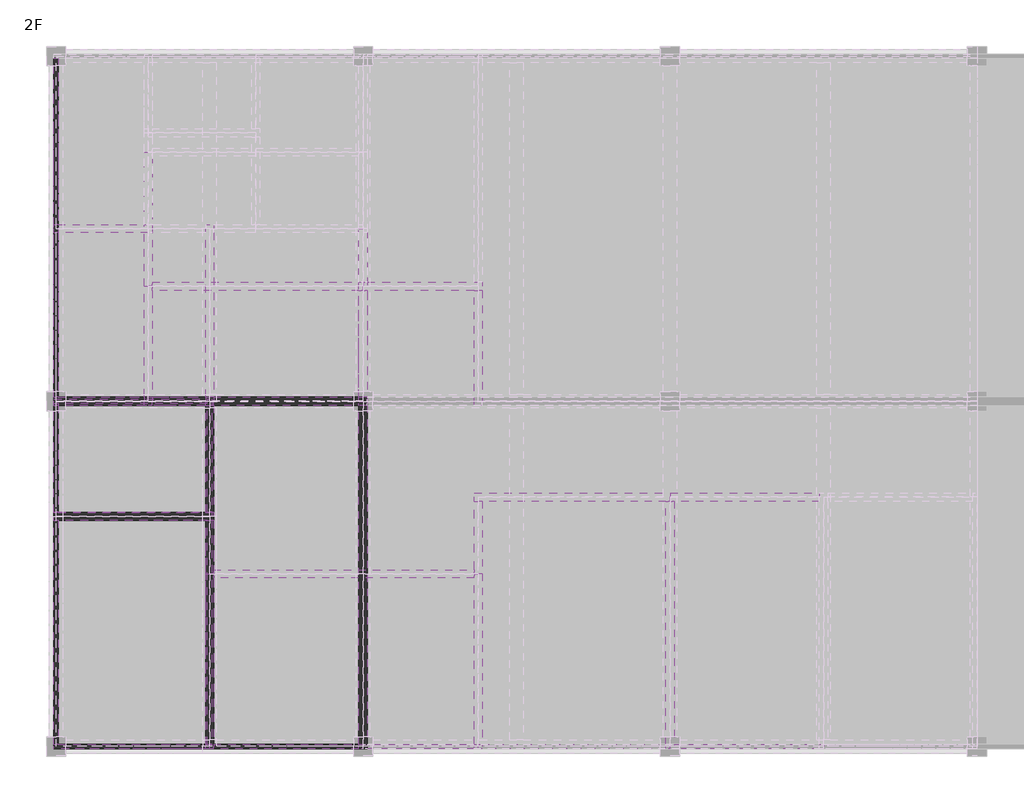
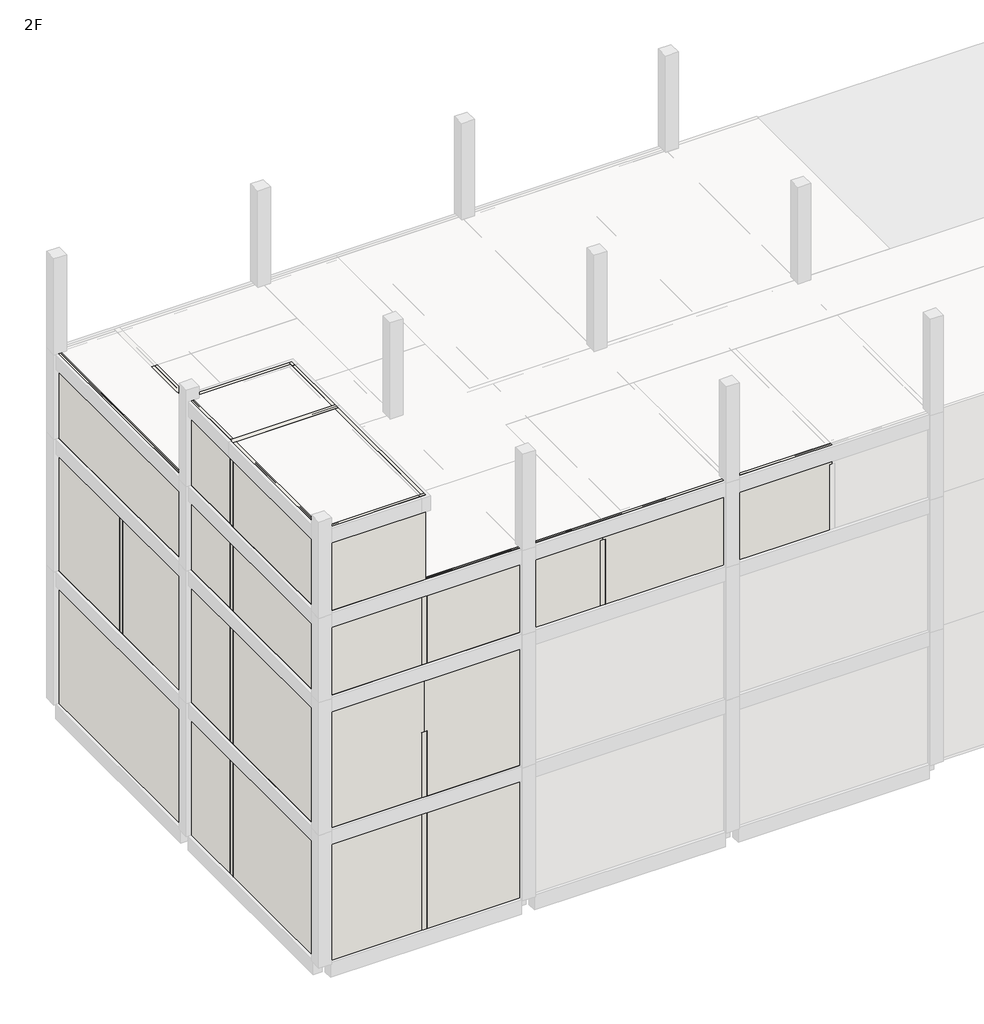
# One storey, part 1 of 7: 58 walls.
# Revit data of these elements (continued)
# Materials (continued)
#   "A04AK073-00001_Concrete Brick_0.5B": class "Concrete", colour RGB 180 180 180, transparency 0, Description = "Conc. Block", W00) Work Master Code = "A04AK073-00001", W01) Work Master_Lv1 = "Finishing Work", W02) Work Master_Lv2 = "Masonry Work", W03) Work Master_Spec.1 = "Concrete Brick", W04) Work Master_Spec.2 = "[0.5B] w/ All Reinf.(Lath, Steel Tie, Anchor Bar, Mortar, ETC.), Filler, Sealant, Lintel/Sill for Opening, ETC.", Cost = 0
#   "A04AS164-00002_Plastering_Int": class "Concrete", colour RGB 183 186 184, transparency 0, Description = "LATEX PAINT ON THK.15 CEMENT PLASTER", W00) Work Master Code = "A04AS164-00002", W01) Work Master_Lv1 = "Finishing Work", W02) Work Master_Lv2 = "Plastering Work", W03) Work Master_Spec.1 = "Plastering", W04) Work Master_Spec.2 = "for Internal Masonry Wall", Cost = 0
#   "A04AL078-00002_Int Wall Painting_Water Emulsion Paint": class "Finish", colour RGB 128 128 64, transparency 0, Description = "Plastic", W00) Work Master Code = "A04AL078-00002", W01) Work Master_Lv1 = "Finishing Work", W02) Work Master_Lv2 = "Painting Work", W03) Work Master_Spec.1 = "Internal Wall Painting", W04) Work Master_Spec.2 = "Water Emulsion Paint", Cost = 0
#   "A04AK069-00002_Reinforced Concrete Block_THK 100-200mm": class "Concrete", colour RGB 180 180 180, transparency 0, Description = "Conc. Block", W00) Work Master Code = "A04AK069-00002", W01) Work Master_Lv1 = "Finishing Work", W02) Work Master_Lv2 = "Masonry Work", W03) Work Master_Spec.1 = "Reinforced Concrete Block", W04) Work Master_Spec.2 = "w/ All Reinf.(Lath, Steel Tie, Anchor Bar, Mortar, ETC.), Filler, Sealant, Lintel/Sill for Opening, ETC.", W05) Work Master_Spec.3 = "100mm<THK≤200mm", Cost = 0
#   "Default Wall": class "Miscellaneous", colour RGB 80 80 80, transparency 0
# Room at (79959.652, 167173.861) mm, phase "New Construction", upper offset 2700 mm, lower offset 0 mm
#   Department = "AR"
#   Base Finish = "WK3"
#   Ceiling Finish = "CL3"
#   Wall Finish = "IW5"
#   Floor Finish = "FL2"
#   Number = "4.5"
#   Name = "Office-1"
#   Interior Finish = "IW5..N/A..N/A,,WK3..N/A,,FL2..N/A,,CL3..N/A"
#   Exterior Finish = "RF1..N/A,,EW2..N/A..N/A"
# Room at (84959.652, 167173.861) mm, phase "New Construction", upper offset 3500 mm, lower offset 0 mm
#   Department = "FF"
#   Base Finish = "WK1"
#   Ceiling Finish = ""
#   Wall Finish = "IW5"
#   Floor Finish = "FL1"
#   Number = "4.6"
#   Name = "Fire Gas Room"
#   Interior Finish = "IW5..N/A..N/A,,WK1..N/A,,FL1..N/A,,N/A..N/A"
#   Exterior Finish = "RF1..N/A,,EW2..N/A..N/A"
# Room at (78709.652, 174423.861) mm, phase "New Construction", upper offset 2700 mm, lower offset 0 mm
#   Department = "AR"
#   Base Finish = "WK3"
#   Ceiling Finish = "CL3"
#   Wall Finish = "IW5"
#   Floor Finish = "FL2"
#   Number = "4.7"
#   Name = "Document Room"
#   Interior Finish = "IW5..N/A..N/A,,WK3..N/A,,FL2..N/A,,CL3..N/A"
#   Exterior Finish = "RF1..N/A,,N/A..N/A..N/A"
# Room at (58959.652, 167173.861) mm, phase "New Construction", upper offset 2700 mm, lower offset 0 mm
#   Department = "AR"
#   Base Finish = "WK3"
#   Ceiling Finish = "CL3"
#   Wall Finish = "IW5"
#   Floor Finish = "FL2"
#   Number = "4.8"
#   Name = "Storage"
#   Interior Finish = "IW5..N/A..N/A,,WK3..N/A,,FL2..N/A,,CL3..N/A"
#   Exterior Finish = "RF1..N/A,,EW1..N/A..N/A"
# Room at (52959.652, 166173.861) mm, phase "New Construction", upper offset 2700 mm, lower offset 0 mm
#   Department = "AR"
#   Base Finish = "WK3"
#   Ceiling Finish = "CL3"
#   Wall Finish = "IW5"
#   Floor Finish = "FL2"
#   Number = "4.9"
#   Name = "Break Room"
#   Interior Finish = "IW5..N/A..N/A,,WK3..N/A,,FL2..N/A,,CL3..N/A"
#   Exterior Finish = "RF1..N/A,,EW2..N/A..N/A"
# Room at (50659.652, 177673.861) mm, phase "New Construction", upper offset 2700 mm, lower offset 0 mm
#   Department = "AR"
#   Base Finish = ""
#   Ceiling Finish = "CL4"
#   Wall Finish = "IW3"
#   Floor Finish = "FL3"
#   Number = "4.10"
#   Name = "Toilet"
#   Interior Finish = "IW3..N/A..N/A,,N/A..N/A,,FL3..N/A,,CL4..N/A"
#   Exterior Finish = "RF1..N/A,,N/A..N/A..N/A"
# Room at (50659.652, 180673.861) mm, phase "New Construction", upper offset 2700 mm, lower offset 0 mm
#   Department = "AR"
#   Base Finish = ""
#   Ceiling Finish = "CL4"
#   Wall Finish = "IW3"
#   Floor Finish = "FL3"
#   Number = "4.11"
#   Name = "Shower"
#   Interior Finish = "IW3..N/A..N/A,,N/A..N/A,,FL3..N/A,,CL4..N/A"
#   Exterior Finish = "RF1..N/A,,EW2..N/A..N/A"
# Room at (61459.652, 177423.861) mm, phase "New Construction", upper offset 5500 mm, lower offset 0 mm
#   Department = "CI"
#   Base Finish = "WK1"
#   Ceiling Finish = "CL1"
#   Wall Finish = "IW5"
#   Floor Finish = "FL1"
#   Number = "2.0"
#   Name = "Electrical Room-1"
#   Interior Finish = "IW5..N/A..N/A,,WK1..N/A,,FL1..N/A,,CL1..N/A"
#   Exterior Finish = "N/A..N/A,,EW1..EW2..N/A"
# Room at (70459.652, 168423.861) mm, phase "New Construction", upper offset 5500 mm, lower offset 0 mm
#   Department = "EL"
#   Base Finish = "WK1"
#   Ceiling Finish = "CL1"
#   Wall Finish = "IW5"
#   Floor Finish = "FL1"
#   Number = "2.1"
#   Name = "Electrical Room-2"
#   Interior Finish = "IW5..N/A..N/A,,WK1..N/A,,FL1..N/A,,CL1..N/A"
#   Exterior Finish = "N/A..N/A,,EW1..EW2..N/A"
# Room at (82459.652, 177423.861) mm, phase "New Construction", upper offset 5500 mm, lower offset 0 mm
#   Department = "AR"
#   Base Finish = "WK1"
#   Ceiling Finish = "CL1"
#   Wall Finish = "IW5"
#   Floor Finish = "FL1"
#   Number = "2.2"
#   Name = "Electrical Room (GIS)"
#   Interior Finish = "IW5..N/A..N/A,,WK1..N/A,,FL1..N/A,,CL1..N/A"
#   Exterior Finish = "N/A..N/A,,EW1..EW2..N/A"
# Room at (51459.652, 168423.861) mm, phase "New Construction", upper offset 2700 mm, lower offset 0 mm
#   Department = "AR"
#   Base Finish = "WK3"
#   Ceiling Finish = "CL3"
#   Wall Finish = "IW5"
#   Floor Finish = "FL2"
#   Number = "2.3"
#   Name = "Lobby"
#   Interior Finish = "IW5..N/A..N/A,,WK3..N/A,,FL2..N/A,,CL3..N/A"
#   Exterior Finish = "N/A..N/A,,EW2..N/A..N/A"
# Room at (47459.652, 171423.861) mm, phase "New Construction", upper offset 5500 mm, lower offset 0 mm
#   Department = "PATHV2"
#   Base Finish = ""
#   Ceiling Finish = ""
#   Wall Finish = ""
#   Floor Finish = ""
#   Number = "2.4"
#   Name = "Elevator"
#   Interior Finish = "N/A..N/A..N/A,,N/A..N/A,,N/A..N/A,,N/A..N/A"
#   Exterior Finish = "N/A..N/A,,EW2..N/A..N/A"
# Room at (47459.652, 166923.861) mm, phase "New Construction", upper offset 5500 mm, lower offset 0 mm
#   Department = "PATHV1"
#   Base Finish = "WK3"
#   Ceiling Finish = "CL1"
#   Wall Finish = "IW5"
#   Floor Finish = "FL2"
#   Number = "2.5"
#   Name = "Staircase"
#   Interior Finish = "IW5..N/A..N/A,,WK3..N/A,,FL2..N/A,,CL1..N/A"
#   Exterior Finish = "N/A..N/A,,EW2..N/A..N/A"
# Room at (65459.652, 177423.861) mm, phase "New Construction", upper offset 3400 mm, lower offset 0 mm
#   Department = "CI"
#   Base Finish = ""
#   Ceiling Finish = "CL3"
#   Wall Finish = "IW5"
#   Floor Finish = "FL5"
#   Number = "3.0"
#   Name = "Central Control Room"
#   Interior Finish = "IW5..N/A..N/A,,N/A..N/A,,FL5..N/A,,CL3..N/A"
#   Exterior Finish = "N/A..N/A,,EW1..N/A..N/A"
# Room at (65459.652, 168423.861) mm, phase "New Construction", upper offset 3000 mm, lower offset 0 mm
#   Department = "CI"
#   Base Finish = ""
#   Ceiling Finish = "CL3"
#   Wall Finish = "IW5"
#   Floor Finish = "FL5"
#   Number = "3.1"
#   Name = "Electronic Room"
#   Interior Finish = "IW5..N/A..N/A,,N/A..N/A,,FL5..N/A,,CL3..N/A"
#   Exterior Finish = "N/A..N/A,,EW1..N/A..N/A"
# Room at (80959.652, 180173.861) mm, phase "New Construction", upper offset 2700 mm, lower offset 0 mm
#   Department = "AR"
#   Base Finish = ""
#   Ceiling Finish = "CL3"
#   Wall Finish = "IW5"
#   Floor Finish = "FL5"
#   Number = "3.2"
#   Name = "Computer Room"
#   Interior Finish = "IW5..N/A..N/A,,N/A..N/A,,FL5..N/A,,CL3..N/A"
#   Exterior Finish = "N/A..N/A,,EW2..N/A..N/A"
# Room at (82459.652, 168423.861) mm, phase "New Construction", upper offset 5500 mm, lower offset 0 mm
#   Department = "EL"
#   Base Finish = ""
#   Ceiling Finish = "CL3"
#   Wall Finish = "IW5"
#   Floor Finish = "FL5"
#   Number = "3.3"
#   Name = "Electrical Room -3"
#   Interior Finish = "IW5..N/A..N/A,,N/A..N/A,,FL5,,CL3..N/A"
#   Exterior Finish = "N/A..N/A,,EW2..N/A..N/A"
# Room at (80959.652, 174673.861) mm, phase "New Construction", upper offset 2700 mm, lower offset 0 mm
#   Department = "CI"
#   Base Finish = ""
#   Ceiling Finish = "CL3"
#   Wall Finish = "IW5"
#   Floor Finish = "FL5"
#   Number = "3.4"
#   Name = "Communication Room"
#   Interior Finish = "IW5..N/A..N/A,,N/A..N/A,,FL5..N/A,,CL3..N/A"
#   Exterior Finish = "N/A..N/A,,N/A..N/A..N/A"
# Room at (46659.652, 179673.861) mm, phase "New Construction", upper offset 5500 mm, lower offset 0 mm
#   Department = "PATHV3"
#   Base Finish = ""
#   Ceiling Finish = ""
#   Wall Finish = ""
#   Floor Finish = ""
#   Number = "3.5"
#   Name = "Duct Shaft"
#   Interior Finish = "N/A..N/A..N/A,,N/A..N/A,,N/A..N/A,,N/A..N/A"
#   Exterior Finish = "N/A..N/A,,EW2..N/A..N/A"
# Room at (47459.652, 175173.861) mm, phase "New Construction", upper offset 2700 mm, lower offset 0 mm
#   Department = "AR"
#   Base Finish = ""
#   Ceiling Finish = "CL4"
#   Wall Finish = "IW3"
#   Floor Finish = "FL3"
#   Number = "3.6"
#   Name = "Toilet (M)"
#   Interior Finish = "IW3..N/A..N/A,,N/A..N/A,,FL3..N/A,,CL4..N/A"
#   Exterior Finish = "N/A..N/A,,EW2..N/A..N/A"
# Room at (52059.652, 179673.861) mm, phase "New Construction", upper offset 2700 mm, lower offset 0 mm
#   Department = "AR"
#   Base Finish = ""
#   Ceiling Finish = "CL4"
#   Wall Finish = "IW3"
#   Floor Finish = "FL3"
#   Number = "3.7"
#   Name = "Toilet"
#   Interior Finish = "IW3..N/A..N/A,,N/A..N/A,,FL3..N/A,,CL4..N/A"
#   Exterior Finish = "N/A..N/A,,EW2..N/A..N/A"
# Room at (49259.652, 180923.861) mm, phase "New Construction", upper offset 2700 mm, lower offset 0 mm
#   Department = "AR"
#   Base Finish = ""
#   Ceiling Finish = "CL4"
#   Wall Finish = "IW3"
#   Floor Finish = "FL3"
#   Number = "3.8"
#   Name = "Shower"
#   Interior Finish = "IW3..N/A..N/A,,N/A..N/A,,FL3..N/A,,CL4..N/A"
#   Exterior Finish = "N/A..N/A,,EW2..N/A..N/A"
# Room at (49259.652, 178673.861) mm, phase "New Construction", upper offset 2700 mm, lower offset 0 mm
#   Department = "AR"
#   Base Finish = "WK3"
#   Ceiling Finish = "CL3"
#   Wall Finish = "IW5"
#   Floor Finish = "FL2"
#   Number = "3.9"
#   Name = "Locker(F)"
#   Interior Finish = "IW5..N/A..N/A,,WK3..N/A,,FL2..N/A,,CL3..N/A"
#   Exterior Finish = "N/A..N/A,,N/A..N/A..N/A"
# Room at (47459.652, 171423.861) mm, phase "New Construction", upper offset 5500 mm, lower offset 0 mm
#   Department = "PATHV2"
#   Base Finish = ""
#   Ceiling Finish = ""
#   Wall Finish = ""
#   Floor Finish = ""
#   Number = "3.10"
#   Name = "Elevator"
#   Interior Finish = "N/A..N/A..N/A,,N/A..N/A,,N/A..N/A,,N/A..N/A"
#   Exterior Finish = "N/A..N/A,,EW2..N/A..N/A"
# Room at (47459.652, 166923.861) mm, phase "New Construction", upper offset 2700 mm, lower offset 0 mm
#   Department = "PATHV1"
#   Base Finish = "WK3"
#   Ceiling Finish = "CL1"
#   Wall Finish = "IW5"
#   Floor Finish = "FL2"
#   Number = "3.11"
#   Name = "Staircase"
#   Interior Finish = "IW5..N/A..N/A,,WK3..N/A,,FL2..N/A,,CL1..N/A"
#   Exterior Finish = "N/A..N/A,,EW2..N/A..N/A"
# Room at (82459.652, 177423.861) mm, phase "New Construction", upper offset 2700 mm, lower offset 0 mm
#   Department = "AR"
#   Base Finish = "WK3"
#   Ceiling Finish = "CL3"
#   Wall Finish = "IW5"
#   Floor Finish = "FL2"
#   Number = "3.12"
#   Name = "Corridor"
#   Interior Finish = "IW5..N/A..N/A,,WK3..N/A,,FL2..N/A,,CL3..N/A"
#   Exterior Finish = "N/A..N/A,,EW2..N/A..N/A"
# Room at (51459.652, 170673.861) mm, phase "New Construction", upper offset 2700 mm, lower offset 0 mm
#   Department = "AR"
#   Base Finish = "WK3"
#   Ceiling Finish = "CL3"
#   Wall Finish = "IW5"
#   Floor Finish = "FL2"
#   Number = "3.13"
#   Name = "Corridor"
#   Interior Finish = "IW5..N/A..N/A,,WK3..N/A,,FL2..N/A,,CL3..N/A"
#   Exterior Finish = "N/A..N/A,,EW2..N/A..N/A"
# Room at (63459.652, 167173.861) mm, phase "New Construction", upper offset 2700 mm, lower offset 0 mm
#   Department = "AR"
#   Base Finish = "WK3"
#   Ceiling Finish = "CL3"
#   Wall Finish = "IW5"
#   Floor Finish = "FL2"
#   Number = "4.0"
#   Name = "Manager Office-1"
#   Interior Finish = "IW5..N/A..N/A,,WK3..N/A,,FL2..N/A,,CL3..N/A"
#   Exterior Finish = "RF1..N/A,,EW1..N/A..N/A"
# Room at (67459.652, 167173.861) mm, phase "New Construction", upper offset 2700 mm, lower offset 0 mm
#   Department = "AR"
#   Base Finish = "WK3"
#   Ceiling Finish = "CL3"
#   Wall Finish = "IW5"
#   Floor Finish = "FL2"
#   Number = "4.1"
#   Name = "Manager Office-2"
#   Interior Finish = "IW5..N/A..N/A,,WK3..N/A,,FL2..N/A,,CL3..N/A"
#   Exterior Finish = "RF1..N/A,,EW1..N/A..N/A"
# Room at (78709.652, 178923.861) mm, phase "New Construction", upper offset 2700 mm, lower offset 0 mm
#   Department = "AR"
#   Base Finish = "WK3"
#   Ceiling Finish = "CL3"
#   Wall Finish = "IW5"
#   Floor Finish = "FL2"
#   Number = "4.2"
#   Name = "Meeting Room-1"
#   Interior Finish = "IW5..N/A..N/A,,WK3..N/A,,FL2..N/A,,CL3..N/A"
#   Exterior Finish = "RF1..N/A,,EW1..EW2..N/A"
# Room at (73459.652, 167173.861) mm, phase "New Construction", upper offset 2700 mm, lower offset 0 mm
#   Department = "AR"
#   Base Finish = "WK3"
#   Ceiling Finish = "CL3"
#   Wall Finish = "IW5"
#   Floor Finish = "FL2"
#   Number = "4.3"
#   Name = "Meeting Room-2"
#   Interior Finish = "IW5..N/A..N/A,,WK3..N/A,,FL2..N/A,,CL3..N/A"
#   Exterior Finish = "RF1..N/A,,EW1..N/A..N/A"
# Room at (64709.652, 177423.861) mm, phase "New Construction", upper offset 2700 mm, lower offset 0 mm
#   Department = "HV"
#   Base Finish = "WK3"
#   Ceiling Finish = "CL3"
#   Wall Finish = "IW5"
#   Floor Finish = "FL2"
#   Number = "4.4"
#   Name = "Open Office"
#   Interior Finish = "IW5..N/A..N/A,,WK3..N/A,,FL2..N/A,,CL3..N/A"
#   Exterior Finish = "RF1..N/A,,EW1..N/A..N/A"
# Room at (54959.652, 178923.861) mm, phase "New Construction", upper offset 2700 mm, lower offset 0 mm
#   Department = "AR"
#   Base Finish = "WK3"
#   Ceiling Finish = "CL3"
#   Wall Finish = "IW5"
#   Floor Finish = "FL2"
#   Number = "4.12"
#   Name = "Locker(M)"
#   Interior Finish = "IW5..N/A..N/A,,WK3..N/A,,FL2..N/A,,CL3..N/A"
#   Exterior Finish = "RF1..N/A,,EW1..N/A..N/A"
# Room at (50659.652, 174423.861) mm, phase "New Construction", upper offset 2700 mm, lower offset 0 mm
#   Department = "AR"
#   Base Finish = ""
#   Ceiling Finish = "CL4"
#   Wall Finish = "IW3"
#   Floor Finish = "FL3"
#   Number = "4.13"
#   Name = "Toilet(F)"
#   Interior Finish = "IW3..N/A..N/A,,N/A..N/A,,FL3..N/A,,CL4..N/A"
#   Exterior Finish = "RF1..N/A,,N/A..N/A..N/A"
# Room at (46659.652, 177423.861) mm, phase "New Construction", upper offset 3500 mm, lower offset 0 mm
#   Department = "PATHV3"
#   Base Finish = ""
#   Ceiling Finish = ""
#   Wall Finish = ""
#   Floor Finish = ""
#   Number = "4.14"
#   Name = "Duct Shaft"
#   Interior Finish = "N/A..N/A..N/A,,N/A..N/A,,N/A..N/A,,N/A..N/A"
#   Exterior Finish = "RF1..N/A,,EW2..N/A..N/A"
# Room at (47459.652, 171423.861) mm, phase "New Construction", upper offset 3500 mm, lower offset 0 mm
#   Department = "PATHV2"
#   Base Finish = ""
#   Ceiling Finish = ""
#   Wall Finish = ""
#   Floor Finish = ""
#   Number = "4.15"
#   Name = "Elevator"
#   Interior Finish = "N/A..N/A..N/A,,N/A..N/A,,N/A..N/A,,N/A..N/A"
#   Exterior Finish = "N/A..N/A,,EW2..N/A..N/A"
# Room at (47459.652, 166923.861) mm, phase "New Construction", upper offset 3500 mm, lower offset 0 mm
#   Department = "PATHV1"
#   Base Finish = ""
#   Ceiling Finish = "CL1"
#   Wall Finish = "IW5"
#   Floor Finish = "FL2"
#   Number = "4.16"
#   Name = "Staircase"
#   Interior Finish = "IW5..N/A..N/A,,N/A..N/A,,FL2..N/A,,CL1..N/A"
#   Exterior Finish = "N/A..N/A,,EW2..N/A..N/A"
# Room at (61397.694, 171673.861) mm, phase "New Construction", upper offset 2700 mm, lower offset 0 mm
#   Department = "AR"
#   Base Finish = "WK3"
#   Ceiling Finish = "CL3"
#   Wall Finish = "IW5"
#   Floor Finish = "FL2"
#   Number = "4.17"
#   Name = "Corridor"
#   Interior Finish = "IW5..N/A..N/A,,WK3..N/A,,FL2..N/A,,CL3..N/A"
#   Exterior Finish = "RF1..N/A,,EW2..N/A..N/A"
# Room at (47459.652, 171423.861) mm, phase "New Construction", upper offset 3500 mm, lower offset 0 mm
#   Department = "PATHV2"
#   Base Finish = ""
#   Ceiling Finish = ""
#   Wall Finish = ""
#   Floor Finish = ""
#   Number = "5.0"
#   Name = "Elevator"
#   Interior Finish = "N/A..N/A..N/A,,N/A..N/A,,N/A..N/A,,N/A..N/A"
#   Exterior Finish = "RF1..N/A,,EW2..EW1..N/A"
# Room at (47459.652, 166923.861) mm, phase "New Construction", upper offset 3500 mm, lower offset 0 mm
#   Department = "PATHV1"
#   Base Finish = "WK3"
#   Ceiling Finish = "CL1"
#   Wall Finish = "IW5"
#   Floor Finish = "FL2"
#   Number = "5.1"
#   Name = "Staircase"
#   Interior Finish = "IW5..N/A..N/A,,WK3..N/A,,FL2..N/A,,CL1..N/A"
#   Exterior Finish = "RF1..N/A,,EW2..EW1..N/A"
